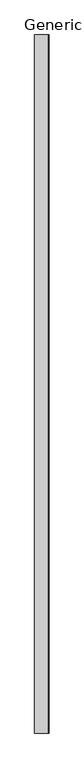
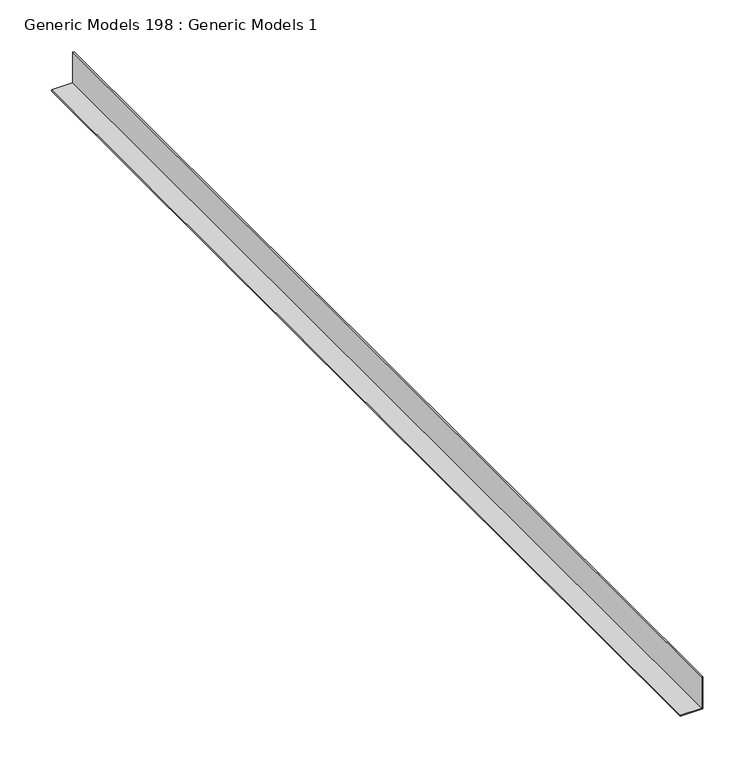
"""IFC4 building model written with IfcOpenShell, lengths in millimetres: proxy geometry, Generic Models 198 : Generic Models 1."""

from ifc_helpers import new_model, si_unit, frame, origin, place, context, project, spatial, polyline, outline, extrude, source, transform, mapped, element, save


def generic_models_198_generic_models_1_ae186574(model_context):
    return source(origin(), model_context, "Body", "SweptSolid", [
        extrude(outline(polyline([(352.6731772, 52542.4946108), (352.6731772, 52540.9071108), (316.1606772, 52540.9071108), (316.1606772, 52517.0946108), (314.5731772, 52517.0946108), (314.5731772, 52542.4946108), (352.6731772, 52542.4946108)])), frame((0.0, 0.0, 0.0), z_axis=(0.0, 1.0, 0.0), x_axis=(0.0, 0.0, 1.0)), (0.0, 0.0, 1.0), 1219.2),
    ])


if __name__ == "__main__":
    model = new_model("IFC4")
    model_context = context("Model", 3, world=origin())
    ifc_project = project(units=[si_unit("LENGTHUNIT", "METRE", prefix="MILLI")], contexts=[model_context])
    site = spatial("IfcSite", under=ifc_project)
    building = spatial("IfcBuilding", under=site)
    placement = place(None, origin())
    generic_models_198_generic_models_1_shape = generic_models_198_generic_models_1_ae186574(model_context)
    element("IfcBuildingElementProxy", 1, Name="Generic Models 198 : Generic Models 1", ObjectType="Generic Models 198 : Generic Models 1", at=placement, inside=building, context=model_context, shape_type="MappedRepresentation", body=[
        mapped(generic_models_198_generic_models_1_shape, transform((0.0, 0.0, 0.0), x_axis=(1.0, 0.0, 0.0), y_axis=(0.0, 1.0, 0.0), z_axis=(0.0, 0.0, 1.0))),
    ])
    save(model, "model.ifc")

# Revit data of these elements
# Element 1 (IfcBuildingElementProxy, "Generic Models 198 : Generic Models 1")
#   Materials on its faces: "CEILING TRACK AS SCHEDULED"
# Materials
#   "CEILING TRACK AS SCHEDULED": class "Unassigned", colour RGB 210 209 208, transparency 0, Keynote = "M05121300.02", Cost = 0
